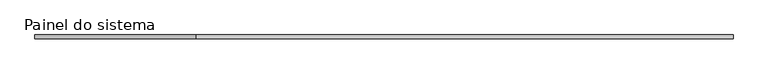
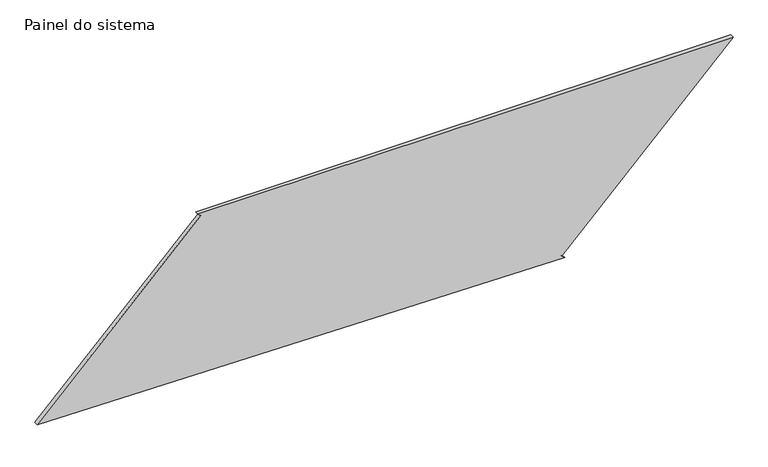
"""IFC4 building model written with IfcOpenShell, lengths in millimetres: plate geometry, Painel do sistema : Envidraçado."""

from ifc_helpers import new_model, si_unit, frame, origin, place, context, project, spatial, polyline, outline, extrude, source, transform, mapped, element, save


def painel_do_sistema_8638cfcf(model_context):
    return source(origin(), model_context, "Body", "SweptSolid", [
        extrude(outline(polyline([(0.0, 1206.4524615), (17.655268, 1188.7524188), (1171.7202199, 2339.8980086), (1171.7202199, -1258.4392747), (1154.0649518, -1240.739232), (52.1186543, -2339.8980086), (0.0, 1206.4524615)])), frame((0.0, 24.5, 0.0), z_axis=(0.0, 1.0, 0.0), x_axis=(0.0, 0.0, 1.0)), (0.0, 0.0, 1.0), 25.0),
    ])


if __name__ == "__main__":
    model = new_model("IFC4")
    model_context = context("Model", 3, world=origin())
    ifc_project = project(units=[si_unit("LENGTHUNIT", "METRE", prefix="MILLI")], contexts=[model_context])
    site = spatial("IfcSite", under=ifc_project)
    building = spatial("IfcBuilding", under=site)
    placement = place(None, origin())
    painel_do_sistema_shape = painel_do_sistema_8638cfcf(model_context)
    element("IfcPlate", 1, ObjectType="Painel do sistema : Envidraçado", at=placement, inside=building, context=model_context, shape_type="MappedRepresentation", body=[
        mapped(painel_do_sistema_shape, transform((0.0, 0.0, 0.0), x_axis=(1.0, 0.0, 0.0), y_axis=(0.0, 1.0, 0.0), z_axis=(0.0, 0.0, 1.0))),
    ])
    save(model, "model.ifc")

# Revit data of these elements
# Type "Painel do sistema : Envidraçado"
#   Construction Type Id = "GSP4R"
#   Analytic Construction = "Vidraça única Pilkington 1/8 pol"
#   Visual Light Transmittance = 0.9
#   Solar Heat Gain Coefficient = 0.86
#   Heat Transfer Coefficient (U) = 6.7069 W/(m²·K)
# Element 1 (IfcPlate, "Painel do sistema : Envidraçado")
#   Materials on its faces: "Vidro"
# Materials
#   "Vidro": class "Vidro", colour RGB 0 128 192, transparency 0.9, Description = "Vidro de sílica", Cost = 0
